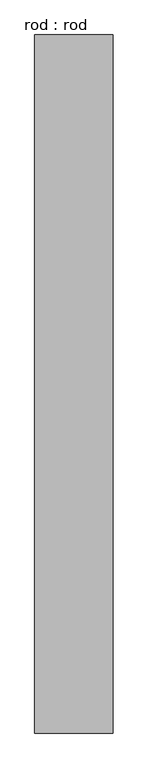
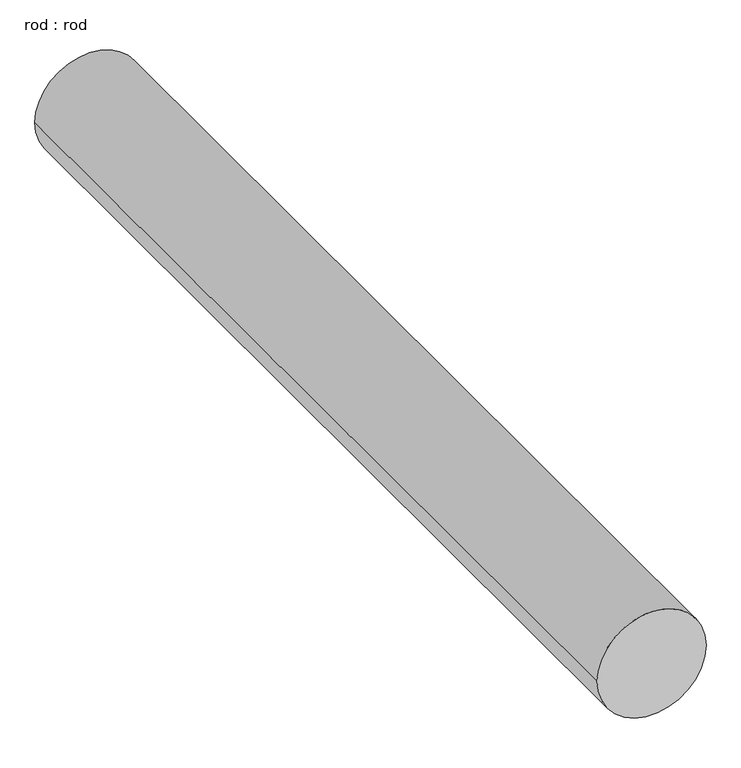
"""IFC4 building model written with IfcOpenShell, lengths in millimetres: proxy geometry, rod : rod."""

from ifc_helpers import new_model, si_unit, point, frame, frame_2d, origin, place, context, project, spatial, circle_curve, trimmed, segment, composite_curve, outline, extrude, source, transform, mapped, element, save


def rod_rod_33b11dd8(model_context):
    return source(origin(), model_context, "Body", "SweptSolid", [
        extrude(outline(composite_curve([segment(trimmed(circle_curve(frame_2d((0.0108462, 0.0)), 200.0), [point((0.0108462, 200.0))], [point((0.0108462, -200.0))], False, "CARTESIAN"), True, "CONTINUOUS"), segment(trimmed(circle_curve(frame_2d((0.0108462, 0.0)), 200.0), [point((0.0108462, -200.0))], [point((0.0108462, 200.0))], False, "CARTESIAN"), True, "CONTINUOUS")], self_intersect=False)), frame((0.0, 2308.0280102, 0.0), z_axis=(0.0, 1.0, 0.0), x_axis=(0.0, 0.0, 1.0)), (0.0, 0.0, 1.0), 3569.4012103),
    ])


if __name__ == "__main__":
    model = new_model("IFC4")
    model_context = context("Model", 3, world=origin())
    ifc_project = project(units=[si_unit("LENGTHUNIT", "METRE", prefix="MILLI")], contexts=[model_context])
    site = spatial("IfcSite", under=ifc_project)
    building = spatial("IfcBuilding", under=site)
    placement = place(None, origin())
    rod_rod_shape = rod_rod_33b11dd8(model_context)
    element("IfcBuildingElementProxy", 1, Name="rod : rod", ObjectType="rod : rod", at=placement, inside=building, context=model_context, shape_type="MappedRepresentation", body=[
        mapped(rod_rod_shape, transform((0.0, 0.0, 0.0), x_axis=(1.0, 0.0, 0.0), y_axis=(0.0, 1.0, 0.0), z_axis=(0.0, 0.0, 1.0))),
    ])
    save(model, "model.ifc")

# Revit data of these elements
# Type "rod : rod"
#   Default Elevation = 0
